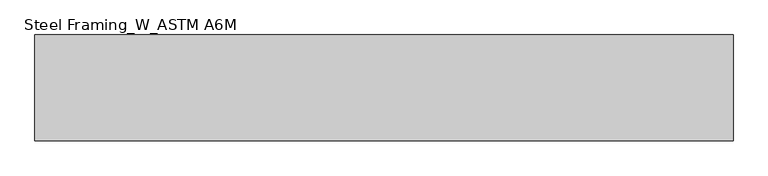
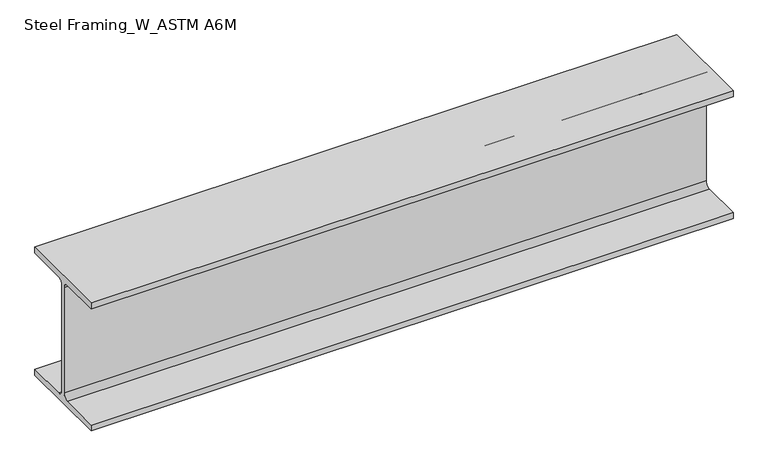
"""IFC4 building model written with IfcOpenShell, lengths in millimetres: beam geometry, Steel Framing_W_ASTM A6M : H_SB_AR_S02_W360x91_CG1."""

from ifc_helpers import new_model, si_unit, point, frame, frame_2d, origin, place, context, project, spatial, polyline, circle_curve, trimmed, segment, composite_curve, outline, extrude, source, transform, mapped, element, save


def steel_framing_w_astm_a6m_3004eec7(model_context):
    return source(origin(), model_context, "Body", "SweptSolid", [
        extrude(outline(composite_curve([segment(polyline([(127.0, -160.1), (127.0, -176.5), (-127.0, -176.5), (-127.0, -160.1), (-19.865, -160.1)]), True, "CONTINUOUS"), segment(trimmed(circle_curve(frame_2d((-19.865, -145.0)), 15.1), [point((-19.865, -160.1))], [point((-4.765, -145.0))], True, "CARTESIAN"), True, "CONTINUOUS"), segment(polyline([(-4.765, -145.0), (-4.765, 145.0)]), True, "CONTINUOUS"), segment(trimmed(circle_curve(frame_2d((-19.865, 145.0)), 15.1), [point((-4.765, 145.0))], [point((-19.865, 160.1))], True, "CARTESIAN"), True, "CONTINUOUS"), segment(polyline([(-19.865, 160.1), (-127.0, 160.1), (-127.0, 176.5), (127.0, 176.5), (127.0, 160.1), (19.865, 160.1)]), True, "CONTINUOUS"), segment(trimmed(circle_curve(frame_2d((19.865, 145.0)), 15.1), [point((19.865, 160.1))], [point((4.765, 145.0))], True, "CARTESIAN"), True, "CONTINUOUS"), segment(polyline([(4.765, 145.0), (4.765, -145.0)]), True, "CONTINUOUS"), segment(trimmed(circle_curve(frame_2d((19.865, -145.0)), 15.1), [point((4.765, -145.0))], [point((19.865, -160.1))], True, "CARTESIAN"), True, "CONTINUOUS"), segment(polyline([(19.865, -160.1), (127.0, -160.1)]), True, "CONTINUOUS")], self_intersect=False)), frame((-696.3, 0.0, 0.0), z_axis=(1.0, 0.0, 0.0), x_axis=(0.0, 1.0, 0.0)), (0.0, 0.0, 1.0), 1673.3),
    ])


if __name__ == "__main__":
    model = new_model("IFC4")
    model_context = context("Model", 3, world=origin())
    ifc_project = project(units=[si_unit("LENGTHUNIT", "METRE", prefix="MILLI")], contexts=[model_context])
    site = spatial("IfcSite", under=ifc_project)
    building = spatial("IfcBuilding", under=site)
    placement = place(None, origin())
    steel_framing_w_astm_a6m_shape = steel_framing_w_astm_a6m_3004eec7(model_context)
    element("IfcBeam", 1, ObjectType="Steel Framing_W_ASTM A6M : H_SB_AR_S02_W360x91_CG1", at=placement, inside=building, context=model_context, shape_type="MappedRepresentation", body=[
        mapped(steel_framing_w_astm_a6m_shape, transform((0.0, 0.0, 0.0), x_axis=(1.0, 0.0, 0.0), y_axis=(0.0, 1.0, 0.0), z_axis=(0.0, 0.0, 1.0))),
    ])
    save(model, "model.ifc")

# Revit data of these elements
# Type "Steel Framing_W_ASTM A6M : H_SB_AR_S02_W360x91_CG1"
#   Type Mark = "CG1"
#   Section Name Key = "W14x61"
#   Width = 25.4 cm
#   Web Thickness = 0.953 cm
#   Web Fillet = 1.51 cm
#   Warping Constant = 1260000.0 cm⁶
#   Torsional Moment of Inertia = 91.20 cm⁴
#   Section Area = 115.0 cm²
#   Plastic Modulus weak axis = 537.0 cm³
#   Plastic Modulus strong axis = 1670.0 cm³
#   Perimeter = 1.68 m²/m
#   Nominal Weight = 91.00 kgf/m
#   Moment of Inertia weak axis = 4450.00 cm⁴
#   Moment of Inertia strong axis = 26600.00 cm⁴
#   Height = 35.3 cm
#   Flange Thickness = 1.64 cm
#   Elastic Modulus weak axis = 352.0 cm³
#   Elastic Modulus strong axis = 1510.0 cm³
#   Centroid Vertical = 17.65 cm
#   Centroid Horizontal = 12.7 cm
#   Length [instance default] = 1500 mm
#   Structural Material [instance default] = Steel, 45-345
#   Bolt Spacing = 0
#   Assembly Code = ""
# Element 1 (IfcBeam, "Steel Framing_W_ASTM A6M : H_SB_AR_S02_W360x91_CG1")
#   Materials on its faces: "Steel, 45-345"
# Materials
#   "Steel, 45-345": class "Metal", colour RGB 189 187 185, transparency 0, Description = "Steel 345 MPa", Cost = 0
